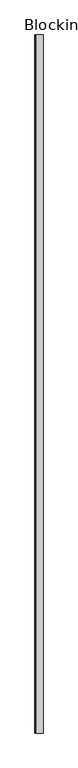
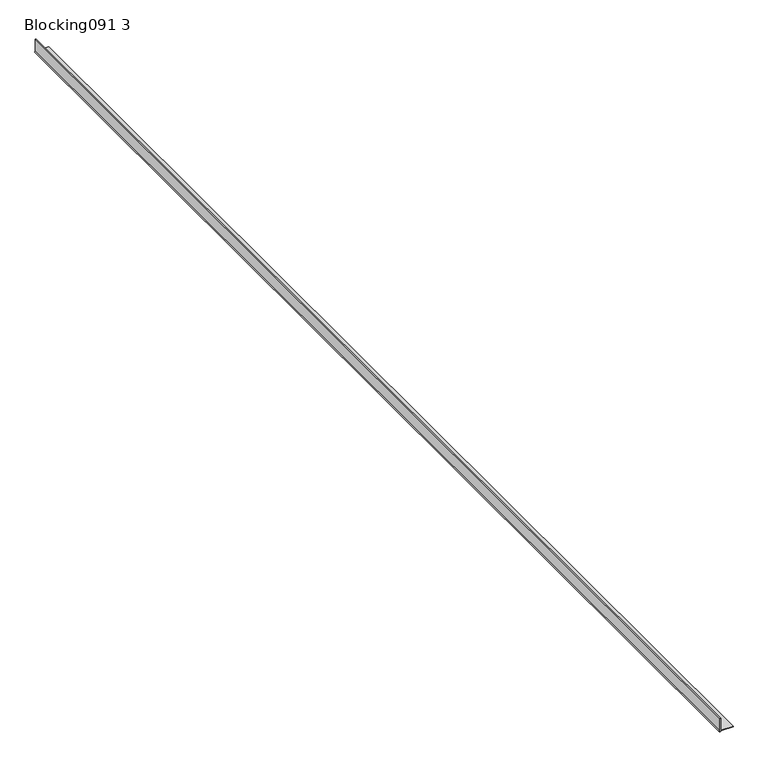
"""IFC4 building model written with IfcOpenShell, lengths in millimetres: proxy geometry, Blocking091 3 : Blocking091 17871."""

from ifc_helpers import new_model, si_unit, point, frame, frame_2d, origin, place, context, project, spatial, polyline, circle_curve, trimmed, segment, composite_curve, outline, extrude, source, transform, mapped, element, save


def blocking091_3_6a2c43f3(model_context):
    return source(origin(), model_context, "Body", "SweptSolid", [
        extrude(outline(composite_curve([segment(polyline([(39579.5041839, 7204.8513569), (39579.5041839, 7203.5713569), (39558.6202421, 7203.5713569)]), True, "CONTINUOUS"), segment(trimmed(circle_curve(frame_2d((39557.3733211, 7203.9204176)), 1.2948572), [point((39558.6202421, 7203.5713569))], [point((39557.071, 7205.1794876))], False, "CARTESIAN"), True, "CONTINUOUS"), segment(polyline([(39557.071, 7205.1794876), (39557.071, 7226.0045408), (39558.351, 7226.0045408), (39558.351, 7204.8513569), (39579.5041839, 7204.8513569)]), True, "CONTINUOUS")], self_intersect=False)), frame((0.0, -3747.9491938, 0.0), z_axis=(0.0, 1.0, 0.0), x_axis=(0.0, 0.0, 1.0)), (0.0, 0.0, 1.0), 2000.0),
    ])


if __name__ == "__main__":
    model = new_model("IFC4")
    model_context = context("Model", 3, world=origin())
    ifc_project = project(units=[si_unit("LENGTHUNIT", "METRE", prefix="MILLI")], contexts=[model_context])
    site = spatial("IfcSite", under=ifc_project)
    building = spatial("IfcBuilding", under=site)
    placement = place(None, origin())
    blocking091_3_shape = blocking091_3_6a2c43f3(model_context)
    element("IfcBuildingElementProxy", 1, Name="Blocking091 3 : Blocking091 17871", ObjectType="Blocking091 3 : Blocking091 17871", at=placement, inside=building, context=model_context, shape_type="MappedRepresentation", body=[
        mapped(blocking091_3_shape, transform((0.0, 0.0, 0.0), x_axis=(1.0, 0.0, 0.0), y_axis=(0.0, 1.0, 0.0), z_axis=(0.0, 0.0, 1.0))),
    ])
    save(model, "model.ifc")

# Revit data of these elements
# Type "Blocking091 3 : Blocking091 17871"
#   NameOverride = "Blocking091"
# Element 1 (IfcBuildingElementProxy, "Blocking091 3 : Blocking091 17871")
#   Materials on its faces: "CORNER BEAD"
# Materials
#   "CORNER BEAD": class "Unassigned", colour RGB 253 236 176, transparency 0, Cost = 0
